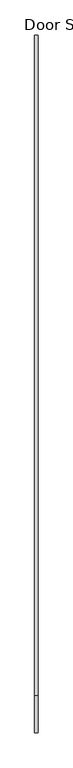
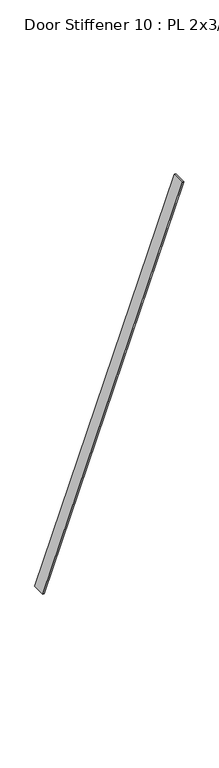
"""IFC4 building model written with IfcOpenShell, lengths in millimetres: proxy geometry, Door Stiffener 10 : PL 2x3/16."""

from ifc_helpers import new_model, si_unit, frame, origin, place, context, project, spatial, polyline, outline, extrude, source, transform, mapped, element, save


def door_stiffener_10_pl_2x3_16_59935e34(model_context):
    return source(origin(), model_context, "Body", "SweptSolid", [
        extrude(outline(polyline([(-536208.5749853, 2400.3), (-535246.0163841, 88.9), (-535301.0452829, 88.9), (-536263.6038841, 2400.3), (-536208.5749853, 2400.3)])), frame((587403.9934739, 0.0, 0.0), z_axis=(1.0, 0.0, 0.0), x_axis=(0.0, 1.0, 0.0)), (0.0, 0.0, 1.0), 4.7625),
    ])


if __name__ == "__main__":
    model = new_model("IFC4")
    model_context = context("Model", 3, world=origin())
    ifc_project = project(units=[si_unit("LENGTHUNIT", "METRE", prefix="MILLI")], contexts=[model_context])
    site = spatial("IfcSite", under=ifc_project)
    building = spatial("IfcBuilding", under=site)
    placement = place(None, origin())
    door_stiffener_10_pl_2x3_16_shape = door_stiffener_10_pl_2x3_16_59935e34(model_context)
    element("IfcBuildingElementProxy", 1, Name="Door Stiffener 10 : PL 2x3/16", ObjectType="Door Stiffener 10 : PL 2x3/16", at=placement, inside=building, context=model_context, shape_type="MappedRepresentation", body=[
        mapped(door_stiffener_10_pl_2x3_16_shape, transform((0.0, 0.0, 0.0), x_axis=(1.0, 0.0, 0.0), y_axis=(0.0, 1.0, 0.0), z_axis=(0.0, 0.0, 1.0))),
    ])
    save(model, "model.ifc")

# Revit data of these elements
# Element 1 (IfcBuildingElementProxy, "Door Stiffener 10 : PL 2x3/16")
#   Materials on its faces: "2\"X3/16\" GALV. STL BAR STOCK"
# Materials
#   "2\"X3/16\" GALV. STL BAR STOCK": class "Generic", colour RGB 211 211 207, transparency 0, Cost = 0
